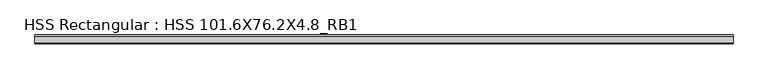
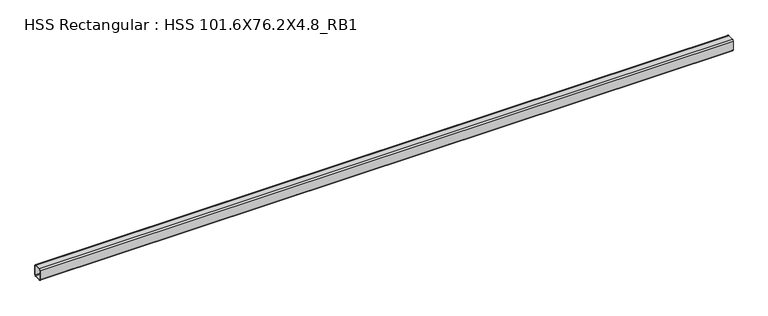
"""IFC4 building model written with IfcOpenShell, lengths in millimetres: beam geometry, HSS Rectangular : HSS 101.6X76.2X4.8_RB1."""

from ifc_helpers import new_model, si_unit, point, frame, frame_2d, origin, place, context, project, spatial, polyline, circle_curve, trimmed, segment, composite_curve, outline, extrude, source, transform, mapped, element, save


def hss_rectangular_hss_101_6x76_2x4_8_rb1_3bb375fb(model_context):
    return source(origin(), model_context, "Body", "SweptSolid", [
        extrude(outline(composite_curve([segment(polyline([(38.1, 41.275), (38.1, -41.275)]), True, "CONTINUOUS"), segment(trimmed(circle_curve(frame_2d((28.575, -41.275)), 9.525), [point((38.1, -41.275))], [point((28.575, -50.8))], False, "CARTESIAN"), True, "CONTINUOUS"), segment(polyline([(28.575, -50.8), (-28.575, -50.8)]), True, "CONTINUOUS"), segment(trimmed(circle_curve(frame_2d((-28.575, -41.275)), 9.525), [point((-28.575, -50.8))], [point((-38.1, -41.275))], False, "CARTESIAN"), True, "CONTINUOUS"), segment(polyline([(-38.1, -41.275), (-38.1, 41.275)]), True, "CONTINUOUS"), segment(trimmed(circle_curve(frame_2d((-28.575, 41.275)), 9.525), [point((-38.1, 41.275))], [point((-28.575, 50.8))], False, "CARTESIAN"), True, "CONTINUOUS"), segment(polyline([(-28.575, 50.8), (28.575, 50.8)]), True, "CONTINUOUS"), segment(trimmed(circle_curve(frame_2d((28.575, 41.275)), 9.525), [point((28.575, 50.8))], [point((38.1, 41.275))], False, "CARTESIAN"), True, "CONTINUOUS")], self_intersect=False), holes=[composite_curve([segment(trimmed(circle_curve(frame_2d((-28.575, 41.275)), 4.7625), [point((-28.575, 46.0375))], [point((-33.3375, 41.275))], True, "CARTESIAN"), True, "CONTINUOUS"), segment(polyline([(-33.3375, 41.275), (-33.3375, -41.275)]), True, "CONTINUOUS"), segment(trimmed(circle_curve(frame_2d((-28.575, -41.275)), 4.7625), [point((-33.3375, -41.275))], [point((-28.575, -46.0375))], True, "CARTESIAN"), True, "CONTINUOUS"), segment(polyline([(-28.575, -46.0375), (28.575, -46.0375)]), True, "CONTINUOUS"), segment(trimmed(circle_curve(frame_2d((28.575, -41.275)), 4.7625), [point((28.575, -46.0375))], [point((33.3375, -41.275))], True, "CARTESIAN"), True, "CONTINUOUS"), segment(polyline([(33.3375, -41.275), (33.3375, 41.275)]), True, "CONTINUOUS"), segment(trimmed(circle_curve(frame_2d((28.575, 41.275)), 4.7625), [point((33.3375, 41.275))], [point((28.575, 46.0375))], True, "CARTESIAN"), True, "CONTINUOUS"), segment(polyline([(28.575, 46.0375), (-28.575, 46.0375)]), True, "CONTINUOUS")], self_intersect=False)]), frame((-7485.254, 0.0, 0.0), z_axis=(1.0, 0.0, 0.0), x_axis=(0.0, 1.0, 0.0)), (0.0, 0.0, 1.0), 5989.111),
    ])


if __name__ == "__main__":
    model = new_model("IFC4")
    model_context = context("Model", 3, world=origin())
    ifc_project = project(units=[si_unit("LENGTHUNIT", "METRE", prefix="MILLI")], contexts=[model_context])
    site = spatial("IfcSite", under=ifc_project)
    building = spatial("IfcBuilding", under=site)
    placement = place(None, origin())
    hss_rectangular_hss_101_6x76_2x4_8_rb1_shape = hss_rectangular_hss_101_6x76_2x4_8_rb1_3bb375fb(model_context)
    element("IfcBeam", 1, ObjectType="HSS Rectangular : HSS 101.6X76.2X4.8_RB1", at=placement, inside=building, context=model_context, shape_type="MappedRepresentation", body=[
        mapped(hss_rectangular_hss_101_6x76_2x4_8_rb1_shape, transform((0.0, 0.0, 0.0), x_axis=(1.0, 0.0, 0.0), y_axis=(0.0, 1.0, 0.0), z_axis=(0.0, 0.0, 1.0))),
    ])
    save(model, "model.ifc")

# Revit data of these elements
# Type "HSS Rectangular : HSS 101.6X76.2X4.8_RB1"
#   Section Name Key = "HSS 4X3X3/16"
#   Assembly Code = "B10"
#   Width = 7.62 cm
#   Wall Nominal Thickness = 0.4763 cm
#   Wall Design Thickness = 0.442 cm
#   Torsional Moment of Inertia = 260.561 cm⁴
#   Torsional Modulus = 61.2876 cm³
#   Section Area = 14.4516 cm²
#   Plastic Modulus weak axis = 40.3122 cm³
#   Plastic Modulus strong axis = 49.1612 cm³
#   Perimeter = 0.881482 m²/m
#   Outer Fillet = 0.9525 cm
#   Nominal Weight = 12.1285 kgf/m
#   Moment of Inertia weak axis = 131.529 cm⁴
#   Moment of Inertia strong axis = 205.202 cm⁴
#   Inner Fillet = 0.4763 cm
#   Height = 10.16 cm
#   Elastic Modulus weak axis = 34.4128 cm³
#   Elastic Modulus strong axis = 40.476 cm³
#   Centroid Vertical = 5.08 cm
#   Centroid Horizontal = 3.81 cm
#   Length [instance default] = 1524 mm
#   Structural Material [instance default] = Steel ASTM A500, Grade B, Rectangular and Square
#   Principal Axes Angle = 0
# Element 1 (IfcBeam, "HSS Rectangular : HSS 101.6X76.2X4.8_RB1")
#   Structural Material = Steel ASTM A992
#   Materials on its faces: "Steel ASTM A992"
# Materials
#   "Steel ASTM A500, Grade B, Rectangular and Square": class "Metal", colour RGB 199 199 199, transparency 0, Description = "Carbon steel", Cost = 0
#   "Steel ASTM A992": class "Metal", colour RGB 199 199 199, transparency 0, Description = "Structural steel 50ksi", Cost = 0
